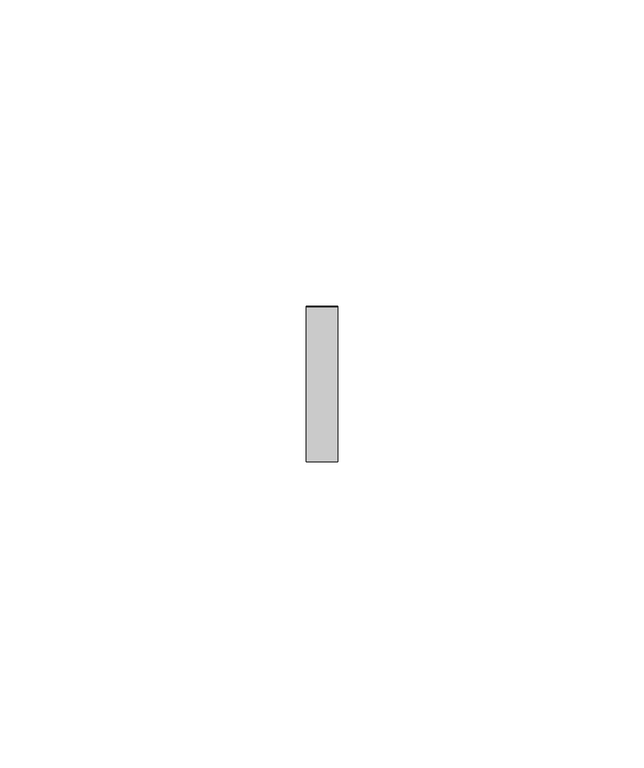
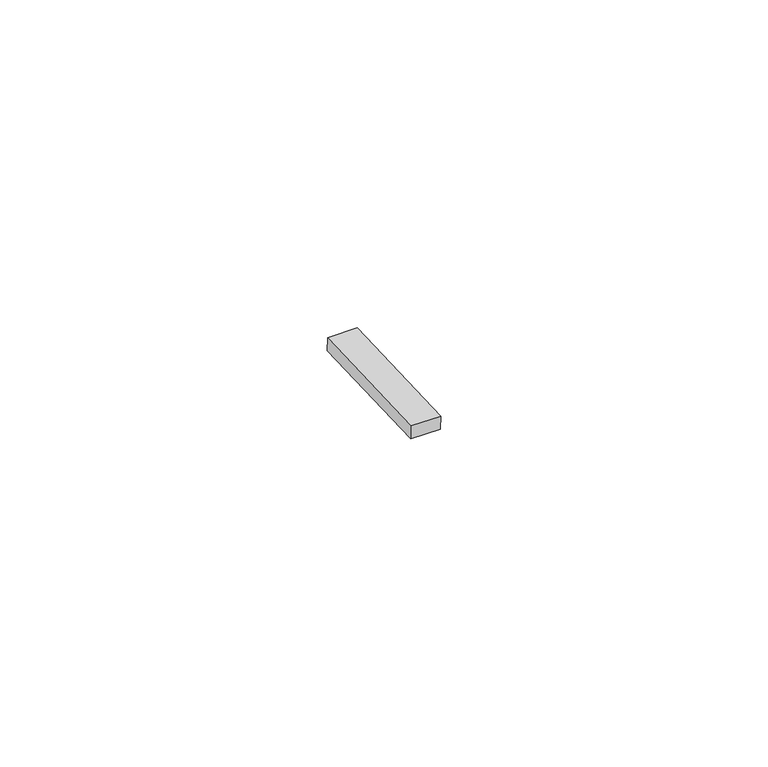
"""IFC4 building model written with IfcOpenShell, lengths in millimetres: proxy geometry, Inner panel:Inner panel:1:Inner panel:1 : Inner panel:Inner panel:300324:2:Inner panel:1:Inner panel:1 : Inner panel:Inner panel:300324:2 : Inner panel:Inner panel:1:Inner panel:1 : Inner panel:Inner panel:300324:300043:132 : Inner panel:Inner panel:1:Inner panel:1 : Inner panel:Inner panel:300324:2:Inner panel:1:Inner panel:1 : Inner panel:Inner panel:300324:2 : Inner panel:Inner panel:1:Inner panel:1 : Inner panel:Inner panel:300324:300043:308120."""

from ifc_helpers import new_model, si_unit, frame, origin, place, context, project, spatial, polyline, outline, extrude, source, transform, mapped, element, save


def generic_models_0a484a24(model_context):
    return source(origin(), model_context, "Body", "SweptSolid", [
        extrude(outline(polyline([(0.0, -25.4), (0.0, 0.0), (5.2138089, 0.0), (5.2138089, -25.4), (0.0, -25.4)])), frame((592310.995117, -576574.3073926, 4050.9976844), z_axis=(0.0, -0.041630544712223896, 0.9991330730923502), x_axis=(-1.0, 0.0, 0.0)), (0.0, 0.0, 1.0), 2.4763745),
    ])


if __name__ == "__main__":
    model = new_model("IFC4")
    model_context = context("Model", 3, world=origin())
    ifc_project = project(units=[si_unit("LENGTHUNIT", "METRE", prefix="MILLI")], contexts=[model_context])
    site = spatial("IfcSite", under=ifc_project)
    building = spatial("IfcBuilding", under=site)
    placement = place(None, origin())
    generic_models_shape = generic_models_0a484a24(model_context)
    element("IfcBuildingElementProxy", 1, Name="Inner panel:Inner panel:1:Inner panel:1 : Inner panel:Inner panel:300324:2:Inner panel:1:Inner panel:1 : Inner panel:Inner panel:300324:2 : Inner panel:Inner panel:1:Inner panel:1 : Inner panel:Inner panel:300324:300043:132 : Inner panel:Inner panel:1:Inner panel:1 : Inner panel:Inner panel:300324:2:Inner panel:1:Inner panel:1 : Inner panel:Inner panel:300324:2 : Inner panel:Inner panel:1:Inner panel:1 : Inner panel:Inner panel:300324:300043:308120", ObjectType="Inner panel:Inner panel:1:Inner panel:1 : Inner panel:Inner panel:300324:2:Inner panel:1:Inner panel:1 : Inner panel:Inner panel:300324:2 : Inner panel:Inner panel:1:Inner panel:1 : Inner panel:Inner panel:300324:300043:132 : Inner panel:Inner panel:1:Inner panel:1 : Inner panel:Inner panel:300324:2:Inner panel:1:Inner panel:1 : Inner panel:Inner panel:300324:2 : Inner panel:Inner panel:1:Inner panel:1 : Inner panel:Inner panel:300324:300043:308120", at=placement, inside=building, context=model_context, shape_type="MappedRepresentation", body=[
        mapped(generic_models_shape, transform((0.0, 0.0, 0.0), x_axis=(1.0, 0.0, 0.0), y_axis=(0.0, 1.0, 0.0), z_axis=(0.0, 0.0, 1.0))),
    ])
    save(model, "model.ifc")

# Revit data of these elements
# Type "Inner panel:Inner panel:1:Inner panel:1 : Inner panel:Inner panel:300324:2:Inner panel:1:Inner panel:1 : Inner panel:Inner panel:300324:2 : Inner panel:Inner panel:1:Inner panel:1 : Inner panel:Inner panel:300324:300043:132 : Inner panel:Inner panel:1:Inner panel:1 : Inner panel:Inner panel:300324:2:Inner panel:1:Inner panel:1 : Inner panel:Inner panel:300324:2 : Inner panel:Inner panel:1:Inner panel:1 : Inner panel:Inner panel:300324:300043:308120"
#   NameOverride = "Inner panel:Inner panel:1:Inner panel:1 : Inner panel:Inner panel:300324:2:Inner panel:1:Inner panel:1 : Inner panel:Inner panel:300324:2 : Inner panel:Inner panel:1:Inner panel:1 : Inner panel:Inner panel:300324:300043:308120"
#   ObjectTypeOverride = "Inner panel:1:Inner panel:1 : Inner panel:Inner panel:300324:2 : Inner panel:Inner panel:1:Inner panel:1 : Inner panel:Inner panel:300324:300043"
#   Reference = "Inner panel"
#   Tag = "308120"
# Element 1 (IfcBuildingElementProxy, "Inner panel:Inner panel:1:Inner panel:1 : Inner panel:Inner panel:300324:2:Inner panel:1:Inner panel:1 : Inner panel:Inner panel:300324:2 : Inner panel:Inner panel:1:Inner panel:1 : Inner panel:Inner panel:300324:300043:132 : Inner panel:Inner panel:1:Inner panel:1 : Inner panel:Inner panel:300324:2:Inner panel:1:Inner panel:1 : Inner panel:Inner panel:300324:2 : Inner panel:Inner panel:1:Inner panel:1 : Inner panel:Inner panel:300324:300043:308120")
#   Materials on its faces: "AT CLIP - 1\" WIDE NON ABSORBENT, WEATHER-RESISTANT NEOPRENE/EPDM/SBR FOAM"
# Materials
#   "AT CLIP - 1\" WIDE NON ABSORBENT, WEATHER-RESISTANT NEOPRENE/EPDM/SBR FOAM": class "Generic", colour RGB 85 85 85, transparency 0, Cost = 0
